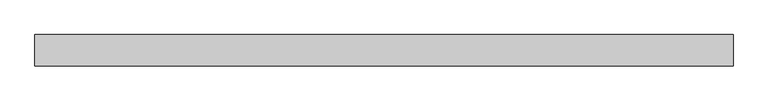
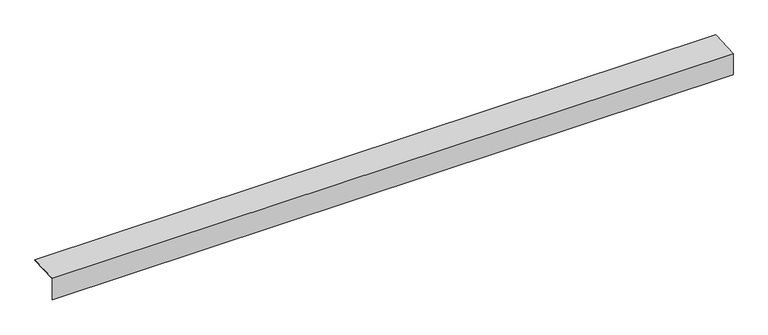
"""IFC4 building model written with IfcOpenShell, lengths in millimetres: proxy geometry, Generic Models 7:Generic Models 1:7:Generic Models 1:7 : Generic Models 7:Generic Models 1:337419:2 : Generic Models 7:Generic Models 1:7:Generic Models 1:7 : Generic Models 7:Generic Models 1:337419:315055."""

from ifc_helpers import new_model, si_unit, frame, origin, place, context, project, spatial, polyline, outline, extrude, source, transform, mapped, element, save


def generic_models_db11356c(model_context):
    return source(origin(), model_context, "Body", "SweptSolid", [
        extrude(outline(polyline([(-579143.2285706, -81.7582633), (-579144.8160706, -81.7582633), (-579144.8160706, -1.1090262), (-579035.2021436, 3.4582208), (-579035.2021436, 1.8693434), (-579143.2285706, -2.6317578), (-579143.2285706, -81.7582633)])), frame((591286.9867239, 0.0, 0.0), z_axis=(1.0, 0.0, 0.0), x_axis=(0.0, 1.0, 0.0)), (0.0, 0.0, 1.0), 2451.1),
    ])


if __name__ == "__main__":
    model = new_model("IFC4")
    model_context = context("Model", 3, world=origin())
    ifc_project = project(units=[si_unit("LENGTHUNIT", "METRE", prefix="MILLI")], contexts=[model_context])
    site = spatial("IfcSite", under=ifc_project)
    building = spatial("IfcBuilding", under=site)
    placement = place(None, origin())
    generic_models_shape = generic_models_db11356c(model_context)
    element("IfcBuildingElementProxy", 1, Name="Generic Models 7:Generic Models 1:7:Generic Models 1:7 : Generic Models 7:Generic Models 1:337419:2 : Generic Models 7:Generic Models 1:7:Generic Models 1:7 : Generic Models 7:Generic Models 1:337419:315055", ObjectType="Generic Models 7:Generic Models 1:7:Generic Models 1:7 : Generic Models 7:Generic Models 1:337419:2 : Generic Models 7:Generic Models 1:7:Generic Models 1:7 : Generic Models 7:Generic Models 1:337419:315055", at=placement, inside=building, context=model_context, shape_type="MappedRepresentation", body=[
        mapped(generic_models_shape, transform((0.0, 0.0, 0.0), x_axis=(1.0, 0.0, 0.0), y_axis=(0.0, 1.0, 0.0), z_axis=(0.0, 0.0, 1.0))),
    ])
    save(model, "model.ifc")

# Revit data of these elements
# Type "Generic Models 7:Generic Models 1:7:Generic Models 1:7 : Generic Models 7:Generic Models 1:337419:2 : Generic Models 7:Generic Models 1:7:Generic Models 1:7 : Generic Models 7:Generic Models 1:337419:315055"
#   NameOverride = "Generic Models 7:Generic Models 1:7:Generic Models 1:7 : Generic Models 7:Generic Models 1:337419:315055"
#   ObjectTypeOverride = "Generic Models 1:7 : Generic Models 7:Generic Models 1:337419"
#   Reference = "Generic Models 1"
#   Tag = "315055"
# Element 1 (IfcBuildingElementProxy, "Generic Models 7:Generic Models 1:7:Generic Models 1:7 : Generic Models 7:Generic Models 1:337419:2 : Generic Models 7:Generic Models 1:7:Generic Models 1:7 : Generic Models 7:Generic Models 1:337419:315055")
#   Materials on its faces: "16 GA. STAINLESS STEEL BRAKE METAL"
# Materials
#   "16 GA. STAINLESS STEEL BRAKE METAL": class "Unassigned", colour RGB 210 209 208, transparency 0, Cost = 0
